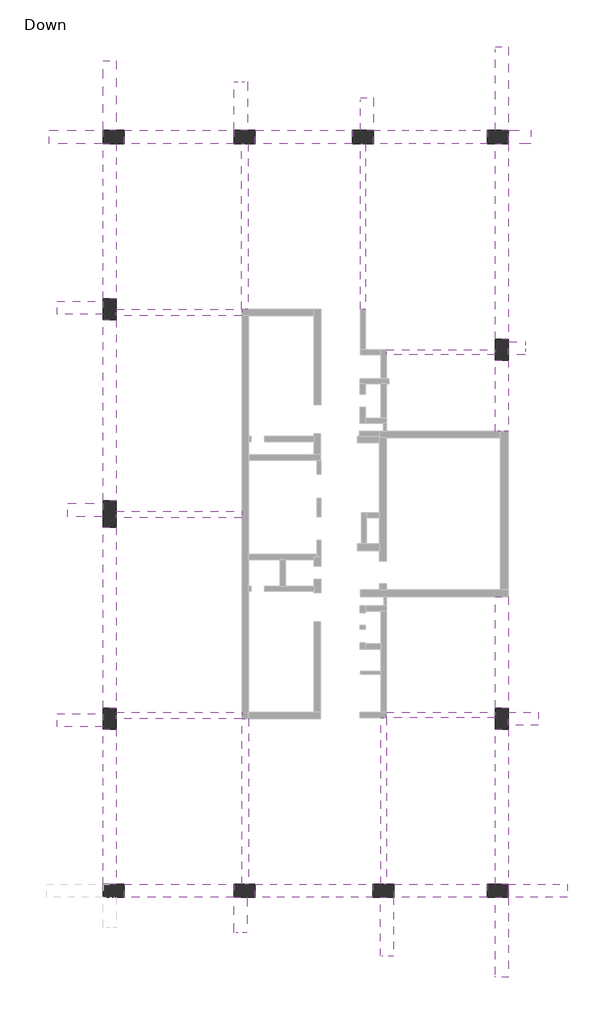
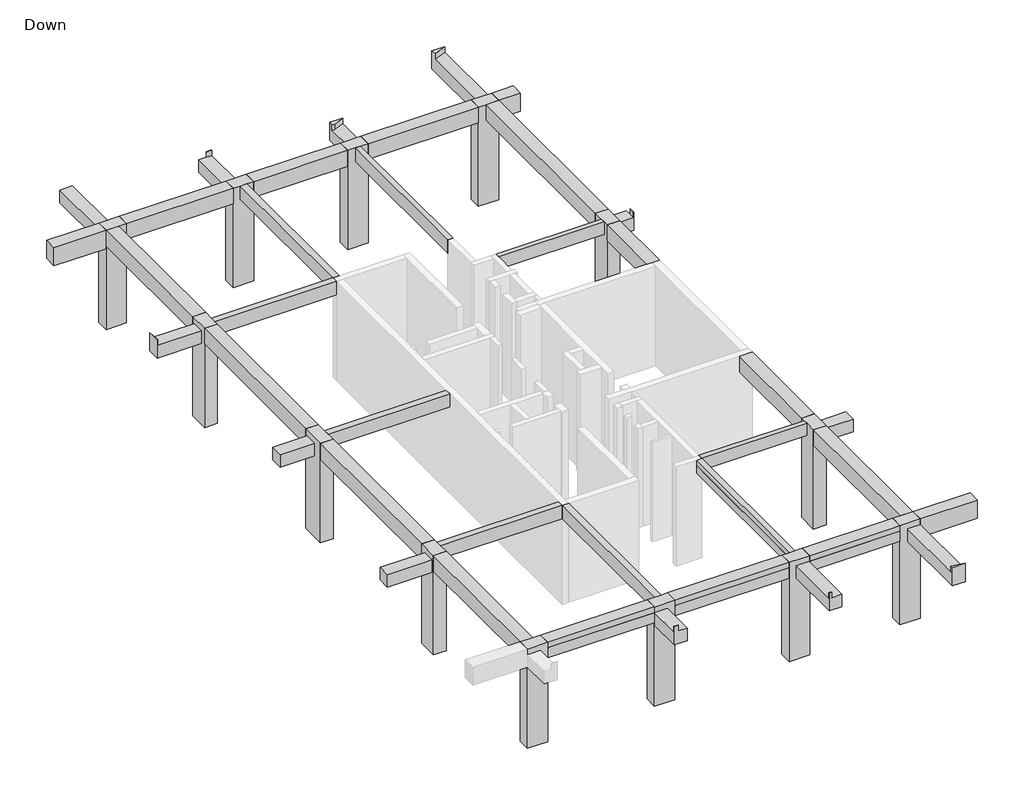
# One storey, part 2 of 2: 38 beams, 13 columns.
# Revit data of these elements (continued)
# Element 39 (IfcColumn, "Concrete Rectengular Column : 50/100")
#   Comments = ""
#   Mark = "C1"
#   SOFiSTiK_AMG_Comments = ""
#   SOFiSTiK_AMG_Scheduled = yes
#   SOFiSTiK_AMG_Adjusted = yes
#   Structural Material = Concrete
#   Phase Created = New Construction
#   Materials on its faces: "Concrete"
# Element 40 (IfcColumn, "Concrete Rectengular Column : 50/80")
#   Comments = ""
#   Mark = "C2"
#   SOFiSTiK_AMG_Comments = ""
#   SOFiSTiK_AMG_Scheduled = yes
#   SOFiSTiK_AMG_Adjusted = yes
#   Structural Material = Concrete
#   Phase Created = New Construction
#   Materials on its faces: "Concrete"
# Element 41 (IfcColumn, "Concrete Rectengular Column : 50/80")
#   Comments = ""
#   Mark = "C3"
#   SOFiSTiK_AMG_Comments = ""
#   SOFiSTiK_AMG_Scheduled = yes
#   SOFiSTiK_AMG_Adjusted = yes
#   Structural Material = Concrete
#   Phase Created = New Construction
#   Materials on its faces: "Concrete"
# Element 42 (IfcColumn, "Concrete Rectengular Column : 50/80")
#   Comments = ""
#   Mark = "C4"
#   SOFiSTiK_AMG_Comments = ""
#   SOFiSTiK_AMG_Scheduled = yes
#   SOFiSTiK_AMG_Adjusted = yes
#   Structural Material = Concrete
#   Phase Created = New Construction
#   Materials on its faces: "Concrete"
# Element 43 (IfcColumn, "Concrete Rectengular Column : 50/80")
#   Comments = ""
#   Mark = "C5"
#   SOFiSTiK_AMG_Comments = ""
#   SOFiSTiK_AMG_Scheduled = yes
#   SOFiSTiK_AMG_Adjusted = yes
#   Structural Material = Concrete
#   Phase Created = New Construction
#   Materials on its faces: "Concrete"
# Element 44 (IfcColumn, "Concrete Rectengular Column : 50/80")
#   Comments = ""
#   Mark = "C6"
#   SOFiSTiK_AMG_Comments = ""
#   SOFiSTiK_AMG_Scheduled = yes
#   SOFiSTiK_AMG_Adjusted = yes
#   Structural Material = Concrete
#   Phase Created = New Construction
#   Materials on its faces: "Concrete"
# Element 45 (IfcColumn, "Concrete Rectengular Column : 50/80")
#   Comments = ""
#   Mark = "C7"
#   SOFiSTiK_AMG_Comments = ""
#   SOFiSTiK_AMG_Scheduled = yes
#   SOFiSTiK_AMG_Adjusted = yes
#   Structural Material = Concrete
#   Phase Created = New Construction
#   Materials on its faces: "Concrete"
# Element 46 (IfcColumn, "Concrete Rectengular Column : 50/80")
#   Comments = ""
#   Mark = "C8"
#   SOFiSTiK_AMG_Comments = ""
#   SOFiSTiK_AMG_Scheduled = yes
#   SOFiSTiK_AMG_Adjusted = yes
#   Structural Material = Concrete
#   Phase Created = New Construction
#   Materials on its faces: "Concrete"
# Element 47 (IfcColumn, "Concrete Rectengular Column : 50/80")
#   Comments = ""
#   Mark = "C9"
#   SOFiSTiK_AMG_Comments = ""
#   SOFiSTiK_AMG_Scheduled = yes
#   SOFiSTiK_AMG_Adjusted = yes
#   Structural Material = Concrete
#   Phase Created = New Construction
#   Materials on its faces: "Concrete"
# Element 48 (IfcColumn, "Concrete Rectengular Column : 50/80")
#   Comments = ""
#   Mark = "C10"
#   SOFiSTiK_AMG_Comments = ""
#   SOFiSTiK_AMG_Scheduled = yes
#   SOFiSTiK_AMG_Adjusted = yes
#   Structural Material = Concrete
#   Phase Created = New Construction
#   Materials on its faces: "Concrete"
# Element 49 (IfcColumn, "Concrete Rectengular Column : 50/80")
#   Comments = ""
#   Mark = "C11"
#   SOFiSTiK_AMG_Comments = ""
#   SOFiSTiK_AMG_Scheduled = yes
#   SOFiSTiK_AMG_Adjusted = yes
#   Structural Material = Concrete
#   Phase Created = New Construction
#   Materials on its faces: "Concrete"
# Element 50 (IfcColumn, "Concrete Rectengular Column : 50/80")
#   Comments = ""
#   Mark = "C12"
#   SOFiSTiK_AMG_Comments = ""
#   SOFiSTiK_AMG_Scheduled = yes
#   SOFiSTiK_AMG_Adjusted = yes
#   Structural Material = Concrete
#   Phase Created = New Construction
#   Materials on its faces: "Concrete"
# Element 51 (IfcColumn, "Concrete Rectengular Column : 50/80")
#   Comments = ""
#   Mark = "C13"
#   SOFiSTiK_AMG_Comments = ""
#   SOFiSTiK_AMG_Scheduled = yes
#   SOFiSTiK_AMG_Adjusted = yes
#   Structural Material = Concrete
#   Phase Created = New Construction
#   Materials on its faces: "Concrete"
# Materials
#   "Concrete": class "Concrete", colour RGB 192 192 192, transparency 0, Keynote = "01000", Description = "Cast-in-place concrete", Cost = 0
